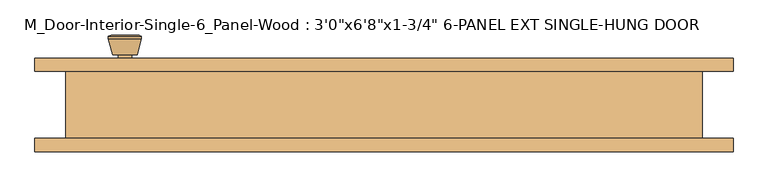
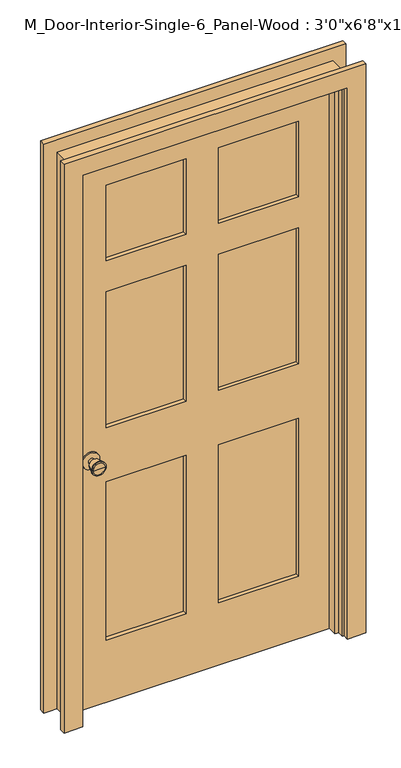
"""IFC4 building model written with IfcOpenShell, lengths in millimetres: door geometry."""

from ifc_helpers import new_model, si_unit, point, frame, frame_2d, origin, place, context, project, spatial, polyline, circle_curve, trimmed, segment, composite_curve, outline, extrude, faceted_brep, source, transform, mapped, element, save
from ifc_brep_helpers import plane_surface, cylinder_surface, revolved_surface, advanced_brep


def door_d838d7c4(model_context):
    return source(origin(), model_context, "Body", "SolidModel", [
        advanced_brep(
        [(-392.2, -2.825, 914.4), (-382.2, -2.825, 914.4), (-402.2, -2.825, 914.4), (-371.7241324, -51.825, 914.4), (-392.2, -51.825, 914.4), (-412.6758676, -51.825, 914.4), (-367.2, -49.9971319, 914.4), (-417.2, -49.9971319, 914.4), (-367.2, -46.5334537, 914.4), (-417.2, -46.5334537, 914.4), (-373.563764, -21.825, 914.4), (-410.836236, -21.825, 914.4), (-382.2, -21.825, 914.4), (-402.2, -21.825, 914.4)],
        [
            (0, 1),
            (1, 2, circle_curve(frame((-392.2, -2.825, 914.4), z_axis=(0.0, 1.0, 0.0), x_axis=(-1.0, 0.0, 0.0)), 10.0)),
            (2, 0),
            (2, 1, circle_curve(frame((-392.2, -2.825, 914.4), z_axis=(0.0, 1.0, 0.0), x_axis=(-1.0, 0.0, 0.0)), 10.0)),
            (3, 4),
            (4, 5),
            (5, 3, circle_curve(frame((-392.2, -51.825, 914.4), z_axis=(0.0, -1.0, 0.0), x_axis=(-1.0, 0.0, 0.0)), 20.4758676)),
            (3, 5, circle_curve(frame((-392.2, -51.825, 914.4), z_axis=(0.0, -1.0, 0.0), x_axis=(-1.0, 0.0, 0.0)), 20.4758676)),
            (6, 3),
            (5, 7),
            (7, 6, circle_curve(frame((-392.2, -49.9971319, 914.4), z_axis=(0.0, -1.0, 0.0), x_axis=(-1.0, 0.0, 0.0)), 25.0)),
            (6, 7, circle_curve(frame((-392.2, -49.9971319, 914.4), z_axis=(0.0, -1.0, 0.0), x_axis=(-1.0, 0.0, 0.0)), 25.0)),
            (8, 6),
            (7, 9),
            (9, 8, circle_curve(frame((-392.2, -46.5334537, 914.4), z_axis=(0.0, -1.0, 0.0), x_axis=(-1.0, 0.0, 0.0)), 25.0)),
            (8, 9, circle_curve(frame((-392.2, -46.5334537, 914.4), z_axis=(0.0, -1.0, 0.0), x_axis=(-1.0, 0.0, 0.0)), 25.0)),
            (10, 8),
            (9, 11),
            (11, 10, circle_curve(frame((-392.2, -21.825, 914.4), z_axis=(0.0, -1.0, 0.0), x_axis=(-1.0, 0.0, 0.0)), 18.636236)),
            (10, 11, circle_curve(frame((-392.2, -21.825, 914.4), z_axis=(0.0, -1.0, 0.0), x_axis=(-1.0, 0.0, 0.0)), 18.636236)),
            (12, 10),
            (11, 13),
            (13, 12, circle_curve(frame((-392.2, -21.825, 914.4), z_axis=(0.0, -1.0, 0.0), x_axis=(-1.0, 0.0, 0.0)), 10.0)),
            (12, 13, circle_curve(frame((-392.2, -21.825, 914.4), z_axis=(0.0, -1.0, 0.0), x_axis=(-1.0, 0.0, 0.0)), 10.0)),
            (1, 12),
            (13, 2),
        ],
        [
            plane_surface(frame((-392.2, -2.825, 914.4), z_axis=(0.0, 1.0, 0.0), x_axis=(-1.0, 0.0, 0.0))),
            plane_surface(frame((-392.2, -51.825, 914.4), z_axis=(0.0, -1.0, 0.0), x_axis=(-1.0, 0.0, 0.0))),
            revolved_surface(polyline([(-412.6758676, -51.825, 914.4), (-417.2, -49.9971319, 914.4)]), (-392.2, -2.825, 914.4), (0.0, 1.0, 0.0)),
            cylinder_surface(frame((-392.2, -2.825, 914.4), z_axis=(0.0, 1.0, 0.0), x_axis=(-1.0, 0.0, 0.0)), 25.0),
            revolved_surface(polyline([(-417.2, -46.5334537, 914.4), (-410.836236, -21.825, 914.4)]), (-392.2, -2.825, 914.4), (0.0, 1.0, 0.0)),
            plane_surface(frame((-392.2, -21.825, 914.4), z_axis=(0.0, 1.0, 0.0), x_axis=(-1.0, 0.0, 0.0))),
            cylinder_surface(frame((-392.2, -2.825, 914.4), z_axis=(0.0, 1.0, 0.0), x_axis=(-1.0, 0.0, 0.0)), 10.0),
        ],
        [
            (0, [[1, 2, 3]]),
            (0, [[-3, 4, -1]]),
            (1, [[5, 6, 7]]),
            (1, [[-6, -5, 8]]),
            (2, [[9, -7, 10, 11]]),
            (2, [[-10, -8, -9, 12]]),
            (3, [[13, -11, 14, 15]]),
            (3, [[-14, -12, -13, 16]]),
            (4, [[17, -15, 18, 19]]),
            (4, [[-18, -16, -17, 20]]),
            (5, [[21, -19, 22, 23]]),
            (5, [[-22, -20, -21, 24]]),
            (6, [[25, -23, 26, -2]]),
            (6, [[-26, -24, -25, -4]]),
        ],
    ),
        extrude(outline(composite_curve([segment(trimmed(circle_curve(frame_2d((914.4, -392.2)), 30.0), [point((914.4, -422.2))], [point((914.4, -362.2))], False, "CARTESIAN"), True, "CONTINUOUS"), segment(trimmed(circle_curve(frame_2d((914.4, -392.2)), 30.0), [point((914.4, -362.2))], [point((914.4, -422.2))], False, "CARTESIAN"), True, "CONTINUOUS")], self_intersect=False)), frame((0.0, -2.825, 0.0), z_axis=(0.0, 1.0, 0.0), x_axis=(0.0, 0.0, 1.0)), (0.0, 0.0, 1.0), 6.0),
        advanced_brep(
        [(-392.2, 53.625, 914.4), (-402.2, 53.625, 914.4), (-382.2, 53.625, 914.4), (-371.7241324, 102.625, 914.4), (-412.6758676, 102.625, 914.4), (-392.2, 102.625, 914.4), (-367.2, 100.7971319, 914.4), (-417.2, 100.7971319, 914.4), (-367.2, 97.3334537, 914.4), (-417.2, 97.3334537, 914.4), (-373.563764, 72.625, 914.4), (-410.836236, 72.625, 914.4), (-382.2, 72.625, 914.4), (-402.2, 72.625, 914.4)],
        [
            (0, 1),
            (1, 2, circle_curve(frame((-392.2, 53.625, 914.4), z_axis=(0.0, -1.0, 0.0), x_axis=(-1.0, 0.0, 0.0)), 10.0)),
            (2, 0),
            (2, 1, circle_curve(frame((-392.2, 53.625, 914.4), z_axis=(0.0, -1.0, 0.0), x_axis=(-1.0, 0.0, 0.0)), 10.0)),
            (3, 4, circle_curve(frame((-392.2, 102.625, 914.4), z_axis=(0.0, 1.0, 0.0), x_axis=(-1.0, 0.0, 0.0)), 20.4758676)),
            (4, 5),
            (5, 3),
            (4, 3, circle_curve(frame((-392.2, 102.625, 914.4), z_axis=(0.0, 1.0, 0.0), x_axis=(-1.0, 0.0, 0.0)), 20.4758676)),
            (6, 7, circle_curve(frame((-392.2, 100.7971319, 914.4), z_axis=(0.0, 1.0, 0.0), x_axis=(-1.0, 0.0, 0.0)), 25.0)),
            (7, 4),
            (3, 6),
            (7, 6, circle_curve(frame((-392.2, 100.7971319, 914.4), z_axis=(0.0, 1.0, 0.0), x_axis=(-1.0, 0.0, 0.0)), 25.0)),
            (8, 9, circle_curve(frame((-392.2, 97.3334537, 914.4), z_axis=(0.0, 1.0, 0.0), x_axis=(-1.0, 0.0, 0.0)), 25.0)),
            (9, 7),
            (6, 8),
            (9, 8, circle_curve(frame((-392.2, 97.3334537, 914.4), z_axis=(0.0, 1.0, 0.0), x_axis=(-1.0, 0.0, 0.0)), 25.0)),
            (10, 11, circle_curve(frame((-392.2, 72.625, 914.4), z_axis=(0.0, 1.0, 0.0), x_axis=(-1.0, 0.0, 0.0)), 18.636236)),
            (11, 9),
            (8, 10),
            (11, 10, circle_curve(frame((-392.2, 72.625, 914.4), z_axis=(0.0, 1.0, 0.0), x_axis=(-1.0, 0.0, 0.0)), 18.636236)),
            (12, 13, circle_curve(frame((-392.2, 72.625, 914.4), z_axis=(0.0, 1.0, 0.0), x_axis=(-1.0, 0.0, 0.0)), 10.0)),
            (13, 11),
            (10, 12),
            (13, 12, circle_curve(frame((-392.2, 72.625, 914.4), z_axis=(0.0, 1.0, 0.0), x_axis=(-1.0, 0.0, 0.0)), 10.0)),
            (1, 13),
            (12, 2),
        ],
        [
            plane_surface(frame((-392.2, 53.625, 914.4), z_axis=(0.0, -1.0, 0.0), x_axis=(-1.0, 0.0, 0.0))),
            plane_surface(frame((-392.2, 102.625, 914.4), z_axis=(0.0, 1.0, 0.0), x_axis=(-1.0, 0.0, 0.0))),
            revolved_surface(polyline([(-412.6758676, 102.625, 914.4), (-417.2, 100.7971319, 914.4)]), (-392.2, 53.625, 914.4), (0.0, -1.0, 0.0)),
            cylinder_surface(frame((-392.2, 53.625, 914.4), z_axis=(0.0, -1.0, 0.0), x_axis=(-1.0, 0.0, 0.0)), 25.0),
            revolved_surface(polyline([(-417.2, 97.3334537, 914.4), (-410.836236, 72.625, 914.4)]), (-392.2, 53.625, 914.4), (0.0, -1.0, 0.0)),
            plane_surface(frame((-392.2, 72.625, 914.4), z_axis=(0.0, -1.0, 0.0), x_axis=(-1.0, 0.0, 0.0))),
            cylinder_surface(frame((-392.2, 53.625, 914.4), z_axis=(0.0, -1.0, 0.0), x_axis=(-1.0, 0.0, 0.0)), 10.0),
        ],
        [
            (0, [[1, 2, 3]]),
            (0, [[-3, 4, -1]]),
            (1, [[5, 6, 7]]),
            (1, [[8, -7, -6]]),
            (2, [[9, 10, -5, 11]]),
            (2, [[12, -11, -8, -10]]),
            (3, [[13, 14, -9, 15]]),
            (3, [[16, -15, -12, -14]]),
            (4, [[17, 18, -13, 19]]),
            (4, [[20, -19, -16, -18]]),
            (5, [[21, 22, -17, 23]]),
            (5, [[24, -23, -20, -22]]),
            (6, [[-2, 25, -21, 26]]),
            (6, [[-4, -26, -24, -25]]),
        ],
    ),
        extrude(outline(composite_curve([segment(trimmed(circle_curve(frame_2d((914.4, -392.2)), 30.0), [point((914.4, -422.2))], [point((914.4, -362.2))], False, "CARTESIAN"), True, "CONTINUOUS"), segment(trimmed(circle_curve(frame_2d((914.4, -392.2)), 30.0), [point((914.4, -362.2))], [point((914.4, -422.2))], False, "CARTESIAN"), True, "CONTINUOUS")], self_intersect=False)), frame((0.0, 47.625, 0.0), z_axis=(0.0, 1.0, 0.0), x_axis=(0.0, 0.0, 1.0)), (0.0, 0.0, 1.0), 6.0),
        extrude(outline(polyline([(337.2, 17.9916667), (57.5, 17.9916667), (57.5, 32.8083333), (337.2, 32.8083333), (337.2, 17.9916667)])), frame((0.0, 0.0, 1632.3), z_axis=(0.0, 0.0, 1.0), x_axis=(1.0, 0.0, 0.0)), (0.0, 0.0, 1.0), 279.7),
        extrude(outline(polyline([(337.2, 17.9916667), (57.5, 17.9916667), (57.5, 32.8083333), (337.2, 32.8083333), (337.2, 17.9916667)])), frame((0.0, 0.0, 1014.4), z_axis=(0.0, 0.0, 1.0), x_axis=(1.0, 0.0, 0.0)), (0.0, 0.0, 1.0), 502.9),
        extrude(outline(polyline([(-57.5, 17.9916667), (-337.2, 17.9916667), (-337.2, 32.8083333), (-57.5, 32.8083333), (-57.5, 17.9916667)])), frame((0.0, 0.0, 1014.4), z_axis=(0.0, 0.0, 1.0), x_axis=(1.0, 0.0, 0.0)), (0.0, 0.0, 1.0), 502.9),
        extrude(outline(polyline([(-57.5, 17.9916667), (-337.2, 17.9916667), (-337.2, 32.8083333), (-57.5, 32.8083333), (-57.5, 17.9916667)])), frame((0.0, 0.0, 1632.3), z_axis=(0.0, 0.0, 1.0), x_axis=(1.0, 0.0, 0.0)), (0.0, 0.0, 1.0), 279.7),
        extrude(outline(polyline([(337.2, 17.9916667), (57.5, 17.9916667), (57.5, 32.8083333), (337.2, 32.8083333), (337.2, 17.9916667)])), frame((0.0, 0.0, 230.0), z_axis=(0.0, 0.0, 1.0), x_axis=(1.0, 0.0, 0.0)), (0.0, 0.0, 1.0), 584.4),
        extrude(outline(polyline([(-57.5, 17.9916667), (-337.2, 17.9916667), (-337.2, 32.8083333), (-57.5, 32.8083333), (-57.5, 17.9916667)])), frame((0.0, 0.0, 230.0), z_axis=(0.0, 0.0, 1.0), x_axis=(1.0, 0.0, 0.0)), (0.0, 0.0, 1.0), 584.4),
        extrude(outline(polyline([(2032.0, -457.2), (0.0, -457.2), (0.0, 457.2), (2032.0, 457.2), (2032.0, -457.2)]), holes=[polyline([(1912.0, 57.5), (1912.0, 337.2), (1632.3, 337.2), (1632.3, 57.5), (1912.0, 57.5)]), polyline([(1517.3, 337.2), (1014.4, 337.2), (1014.4, 57.5), (1517.3, 57.5), (1517.3, 337.2)]), polyline([(1014.4, -57.5), (1014.4, -337.2), (1517.3, -337.2), (1517.3, -57.5), (1014.4, -57.5)]), polyline([(1632.3, -337.2), (1912.0, -337.2), (1912.0, -57.5), (1632.3, -57.5), (1632.3, -337.2)]), polyline([(814.4, 57.5), (814.4, 337.2), (230.0, 337.2), (230.0, 57.5), (814.4, 57.5)]), polyline([(230.0, -57.5), (230.0, -337.2), (814.4, -337.2), (814.4, -57.5), (230.0, -57.5)])]), frame((0.0, 3.175, 0.0), z_axis=(0.0, 1.0, 0.0), x_axis=(0.0, 0.0, 1.0)), (0.0, 0.0, 1.0), 44.45),
        faceted_brep([(482.2, 47.625, 0.0), (482.2, -53.975, 0.0), (457.2, -53.975, 0.0), (457.2, -31.75, 0.0), (444.5, -31.75, 0.0), (444.5, 3.175, 0.0), (457.2, 3.175, 0.0), (457.2, 47.625, 0.0), (482.2, 47.625, 2057.0), (482.2, -53.975, 2057.0), (-482.2, -53.975, 2057.0), (-482.2, -53.975, 0.0), (-457.2, -53.975, 0.0), (-457.2, -53.975, 2032.0), (457.2, -53.975, 2032.0), (457.2, -31.75, 2032.0), (-457.2, -31.75, 2032.0), (-457.2, -31.75, 0.0), (-444.5, -31.75, 0.0), (-444.5, -31.75, 2019.3), (444.5, -31.75, 2019.3), (444.5, 3.175, 2019.3), (-444.5, 3.175, 2019.3), (-444.5, 3.175, 0.0), (-457.2, 3.175, 0.0), (-457.2, 3.175, 2032.0), (457.2, 3.175, 2032.0), (457.2, 47.625, 2032.0), (-457.2, 47.625, 2032.0), (-457.2, 47.625, 0.0), (-482.2, 47.625, 0.0), (-482.2, 47.625, 2057.0)], [[[0, 1, 2, 3, 4, 5, 6, 7]], [[1, 0, 8, 9]], [[2, 1, 9, 10, 11, 12, 13, 14]], [[3, 2, 14, 15]], [[4, 3, 15, 16, 17, 18, 19, 20]], [[5, 4, 20, 21]], [[6, 5, 21, 22, 23, 24, 25, 26]], [[7, 6, 26, 27]], [[0, 7, 27, 28, 29, 30, 31, 8]], [[9, 8, 31, 10]], [[15, 14, 13, 16]], [[21, 20, 19, 22]], [[27, 26, 25, 28]], [[30, 29, 24, 23, 18, 17, 12, 11]], [[10, 31, 30, 11]], [[16, 13, 12, 17]], [[22, 19, 18, 23]], [[28, 25, 24, 29]]]),
        extrude(outline(polyline([(0.0, 463.55), (0.0, 528.55), (2103.35, 528.55), (2103.35, -528.55), (0.0, -528.55), (0.0, -463.55), (2038.35, -463.55), (2038.35, 463.55), (0.0, 463.55)])), frame((0.0, -73.975, 0.0), z_axis=(0.0, 1.0, 0.0), x_axis=(0.0, 0.0, 1.0)), (0.0, 0.0, 1.0), 20.0),
        extrude(outline(polyline([(0.0, 463.55), (0.0, 528.55), (2103.35, 528.55), (2103.35, -528.55), (0.0, -528.55), (0.0, -463.55), (2038.35, -463.55), (2038.35, 463.55), (0.0, 463.55)])), frame((0.0, 47.625, 0.0), z_axis=(0.0, 1.0, 0.0), x_axis=(0.0, 0.0, 1.0)), (0.0, 0.0, 1.0), 20.0),
    ])


if __name__ == "__main__":
    model = new_model("IFC4")
    model_context = context("Model", 3, world=origin())
    ifc_project = project(units=[si_unit("LENGTHUNIT", "METRE", prefix="MILLI")], contexts=[model_context])
    site = spatial("IfcSite", under=ifc_project)
    building = spatial("IfcBuilding", under=site)
    placement = place(None, origin())
    door_shape = door_d838d7c4(model_context)
    element("IfcDoor", 1, ObjectType="M_Door-Interior-Single-6_Panel-Wood : 3'0\"x6'8\"x1-3/4\" 6-PANEL EXT SINGLE-HUNG DOOR", at=placement, inside=building, context=model_context, shape_type="MappedRepresentation", body=[
        mapped(door_shape, transform((0.0, 0.0, 0.0), x_axis=(1.0, 0.0, 0.0), y_axis=(0.0, 1.0, 0.0), z_axis=(0.0, 0.0, 1.0))),
    ])
    save(model, "model.ifc")

# Revit data of these elements
# Type "M_Door-Interior-Single-6_Panel-Wood : 3'0\"x6'8\"x1-3/4\" 6-PANEL EXT SINGLE-HUNG DOOR"
#   Type Mark = "38"
#   Assembly Code = "C1020300"
#   Analytic Construction = "Wooden"
#   Top Rail = 0' - 4.72441"
#   Top Panel = 0' - 11.01181"
#   Thickness = 0' - 1 3/4"
#   Thermal Resistance (R) = 2.5876 (h·ft²·°F)/BTU
#   Swing Angle [instance default] = 90.00°
#   Stiles = 0' - 4.72441"
#   Rough Width = 3' - 1.9685"
#   Rough Height = 6' - 8.98425"
#   Mullion = 0' - 4.52756"
#   Lock Rail = 0' - 7.87402"
#   Intermediate Rail = 0' - 4.52756"
#   Height = 6' - 8"
#   Width = 3' - 0"
#   Heat Transfer Coefficient (U) = 0.3865 BTU/(h·ft²·°F)
#   Bottom Rail = 0' - 9.05512"
#   Trim Material = Cherry
#   Panel Material = Cherry
#   Frame Material = Cherry
#   Door Handle Material = Aluminum
#   Visual Light Transmittance = 0
#   Solar Heat Gain Coefficient = 0
#   Wall Closure = (empty or 0)
#   Function = (empty or 0)
# Element 1 (IfcDoor, "M_Door-Interior-Single-6_Panel-Wood : 3'0\"x6'8\"x1-3/4\" 6-PANEL EXT SINGLE-HUNG DOOR")
#   Materials on its faces: "Cherry", "Aluminum"
# Materials
#   "Cherry": class "Wood", colour RGB 226 177 128, transparency 0, Description = "Prunus Serotina", Cost = 0
#   "Aluminum": class "Metal", colour RGB 244 244 244, transparency 0, Description = "Aluminum 6061", Cost = 0
